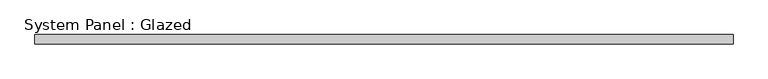
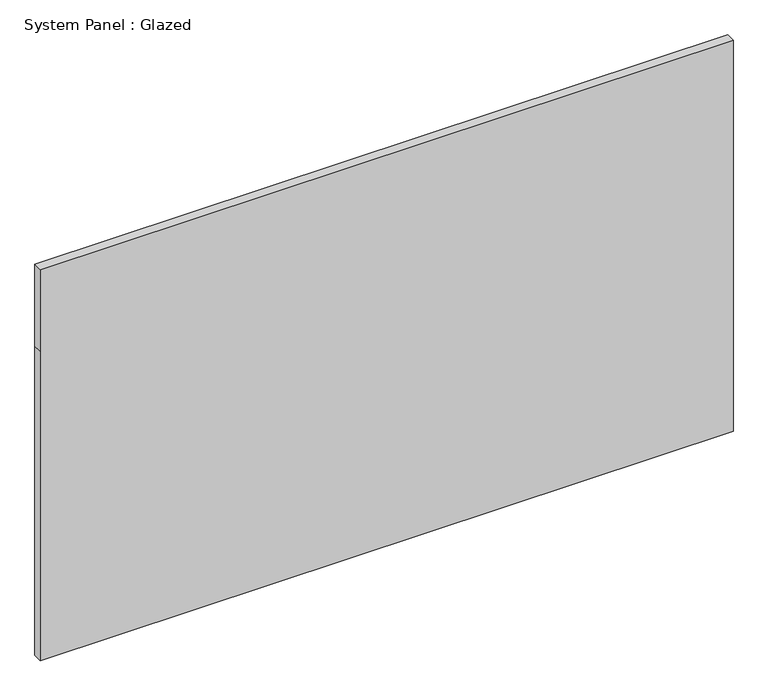
"""IFC4 building model written with IfcOpenShell, lengths in millimetres: plate geometry, System Panel : Glazed."""

import ifcopenshell
import ifcopenshell.guid

model = None  # the IFC model being written
_history = None  # IfcOwnerHistory: only IFC2X3 demands one
_inside = {}  # id of a spatial element -> (the spatial element, [elements in it])
_under = {}  # id of a project, library or spatial element -> (it, [spatial elements below it])
_declared = {}  # id of a project -> (the project, [libraries it declares])
_typed = {}  # id of a type object -> (the type object, [elements of that type])
_made_of = {}  # id of a material, layer set ... -> (it, [elements and type objects made of it])


def new_model(schema):
    """Start an empty IFC model of exactly this schema.

    Asked for "IFC4X3", IfcOpenShell would pick the latest addendum, in which some entities
    have other attributes; the version numbers below select the first issue.
    IFC2X3 requires an IfcOwnerHistory on every rooted entity: one is made here for all.
    """
    global model, _history
    if schema == "IFC4X3":
        model = ifcopenshell.file(schema_version=(4, 3, 0, 0))
    else:
        model = ifcopenshell.file(schema=schema)
    _inside.clear()
    _under.clear()
    _declared.clear()
    _typed.clear()
    _made_of.clear()
    _history = None
    if model.schema == "IFC2X3":
        org = make("IfcOrganization", Name="unknown")
        user = make(
            "IfcPersonAndOrganization",
            ThePerson=make("IfcPerson", FamilyName="unknown"),
            TheOrganization=org,
        )
        app = make(
            "IfcApplication",
            ApplicationDeveloper=org,
            Version="unknown",
            ApplicationFullName="unknown",
            ApplicationIdentifier="unknown",
        )
        _history = make(
            "IfcOwnerHistory",
            OwningUser=user,
            OwningApplication=app,
            ChangeAction="ADDED",
            CreationDate=0,
        )
    return model


def make(cls, **values):
    """One entity of the class cls with the attributes given. An attribute that is None is left unset."""
    return model.create_entity(
        cls, **{name: value for name, value in values.items() if value is not None}
    )


def rooted(cls, **values):
    """An entity with a GlobalId (a new one), such as an element, a storey or a relation."""
    return make(cls, GlobalId=ifcopenshell.guid.new(), OwnerHistory=_history, **values)


def si_unit(unit_type, name, prefix=None):
    """IfcSIUnit, for example si_unit("LENGTHUNIT", "METRE", prefix="MILLI")."""
    return make("IfcSIUnit", UnitType=unit_type, Prefix=prefix, Name=name)


def assignment(units):
    """IfcUnitAssignment: the units of a project."""
    return None if units is None else make("IfcUnitAssignment", Units=units)


def point(xyz):
    """IfcCartesianPoint."""
    return None if xyz is None else make("IfcCartesianPoint", Coordinates=xyz)


def direction(xyz):
    """IfcDirection."""
    return None if xyz is None else make("IfcDirection", DirectionRatios=xyz)


def frame(location, z_axis=None, x_axis=None):
    """IfcAxis2Placement3D, a coordinate frame: its origin and axes. An axis left out is left unset."""
    return make(
        "IfcAxis2Placement3D",
        Location=point(location),
        Axis=direction(z_axis),
        RefDirection=direction(x_axis),
    )


def origin():
    """The frame at (0, 0, 0) with its axes left unset."""
    return frame((0.0, 0.0, 0.0))


def place(relative_to, where):
    """IfcLocalPlacement: puts the frame where relative to a parent placement (None: the world)."""
    return make(
        "IfcLocalPlacement", PlacementRelTo=relative_to, RelativePlacement=where
    )


def context(
    kind, dimensions, precision=None, world=None, true_north=None, identifier=None
):
    """IfcGeometricRepresentationContext, for example the 3D "Model" context."""
    return make(
        "IfcGeometricRepresentationContext",
        ContextIdentifier=identifier,
        ContextType=kind,
        CoordinateSpaceDimension=dimensions,
        Precision=precision,
        WorldCoordinateSystem=world,
        TrueNorth=true_north,
    )


def project(units=None, contexts=None):
    """IfcProject with its units and contexts."""
    return rooted(
        "IfcProject",
        Name="project",
        RepresentationContexts=contexts,
        UnitsInContext=assignment(units),
    )


def spatial(cls, under=None, at=None, **own):
    """A site, building, storey or space (cls), placed at a placement, below another one or the project."""
    s = rooted(cls, ObjectPlacement=at, **own)
    if under is not None:
        _under.setdefault(under.id(), (under, []))[1].append(s)
    return s


def polyline(points):
    """IfcPolyline through the points."""
    return make("IfcPolyline", Points=[point(p) for p in points])


def outline(outer, holes=None, kind="AREA"):
    """IfcArbitraryClosedProfileDef: a profile drawn as a closed curve; with holes, ...WithVoids."""
    if holes is None:
        return make("IfcArbitraryClosedProfileDef", ProfileType=kind, OuterCurve=outer)
    return make(
        "IfcArbitraryProfileDefWithVoids",
        ProfileType=kind,
        OuterCurve=outer,
        InnerCurves=holes,
    )


def extrude(swept, where, along, depth):
    """IfcExtrudedAreaSolid: the profile swept, set in the frame where, extruded along a direction by depth."""
    return make(
        "IfcExtrudedAreaSolid",
        SweptArea=swept,
        Position=where,
        ExtrudedDirection=direction(along),
        Depth=depth,
    )


def shape(context_of_items, identifier, shape_type, items):
    """IfcShapeRepresentation: the items that make up one representation, for example the "Body"."""
    return make(
        "IfcShapeRepresentation",
        ContextOfItems=context_of_items,
        RepresentationIdentifier=identifier,
        RepresentationType=shape_type,
        Items=items,
    )


def source(mapping_origin, context_of_items, identifier, shape_type, items):
    """IfcRepresentationMap: a shape defined once, which mapped items show again and again."""
    return make(
        "IfcRepresentationMap",
        MappingOrigin=mapping_origin,
        MappedRepresentation=shape(context_of_items, identifier, shape_type, items),
    )


def transform(
    local_origin,
    x_axis=None,
    y_axis=None,
    z_axis=None,
    scale=None,
    scale2=None,
    scale3=None,
    uniform=True,
):
    """IfcCartesianTransformationOperator3D, or its non-uniform kind. x_axis, y_axis, z_axis: its Axis1, 2, 3."""
    if uniform:
        return make(
            "IfcCartesianTransformationOperator3D",
            Axis1=direction(x_axis),
            Axis2=direction(y_axis),
            LocalOrigin=point(local_origin),
            Scale=scale,
            Axis3=direction(z_axis),
        )
    return make(
        "IfcCartesianTransformationOperator3DnonUniform",
        Axis1=direction(x_axis),
        Axis2=direction(y_axis),
        LocalOrigin=point(local_origin),
        Scale=scale,
        Axis3=direction(z_axis),
        Scale2=scale2,
        Scale3=scale3,
    )


def mapped(mapping_source, mapping_target):
    """IfcMappedItem: shows the shape of a source again, moved by a transform."""
    return make(
        "IfcMappedItem", MappingSource=mapping_source, MappingTarget=mapping_target
    )


def made_of(thing, what):
    """Note that an element or type object is made of a material, layer set ...; save() writes the relation."""
    if what is not None:
        _made_of.setdefault(what.id(), (what, []))[1].append(thing)
    return thing


def element(
    cls,
    number,
    at=None,
    inside=None,
    cuts=None,
    type_object=None,
    material=None,
    context=None,
    identifier="Body",
    shape_type=None,
    held_by="IfcProductDefinitionShape",
    body=None,
    shapes=None,
    **own,
):
    """One element of the class cls, such as IfcWall. Its Tag is "e" and its number.

    at: its placement. inside: the storey or other place that contains it. cuts: it is an
    opening in that element (IfcRelVoidsElement). A single representation is given by context,
    identifier, shape_type and body (its items); several are given by shapes. held_by: the class
    of the entity that holds the representations. save() writes the other relations.
    """
    e = rooted(cls, Tag="e%d" % number, ObjectPlacement=at, **own)
    if body is not None:
        shapes = [shape(context, identifier, shape_type, body)]
    if shapes is not None:
        e.Representation = make(held_by, Representations=shapes)
    if inside is not None:
        _inside.setdefault(inside.id(), (inside, []))[1].append(e)
    if cuts is not None:
        rooted(
            "IfcRelVoidsElement", RelatingBuildingElement=cuts, RelatedOpeningElement=e
        )
    if type_object is not None:
        _typed.setdefault(type_object.id(), (type_object, []))[1].append(e)
    return made_of(e, material)


def aggregate(whole, parts):
    """IfcRelAggregates: a whole, such as a stair, and the parts it consists of."""
    return rooted("IfcRelAggregates", RelatingObject=whole, RelatedObjects=parts)


def save(model, path):
    """Write the relations noted so far, then the file.

    IfcRelAggregates (storeys below a building ...), IfcRelContainedInSpatialStructure (elements
    in a storey), IfcRelDefinesByType, IfcRelAssociatesMaterial and IfcRelDeclares: one each for
    every whole, place, type object, material and project.
    """
    for whole, parts in _under.values():
        aggregate(whole, parts)
    for where, things in _inside.values():
        rooted(
            "IfcRelContainedInSpatialStructure",
            RelatedElements=things,
            RelatingStructure=where,
        )
    for kind, things in _typed.values():
        rooted("IfcRelDefinesByType", RelatedObjects=things, RelatingType=kind)
    for what, things in _made_of.values():
        rooted("IfcRelAssociatesMaterial", RelatedObjects=things, RelatingMaterial=what)
    for by, libraries in _declared.values():
        rooted("IfcRelDeclares", RelatingContext=by, RelatedDefinitions=libraries)
    model.write(path)


def system_panel_glazed_d60e1f89(model_context):
    return source(origin(), model_context, "Body", "SweptSolid", [
        extrude(outline(polyline([(0.0, -968.375), (0.0, 968.375), (914.4, 968.375), (1155.7, 968.375), (1155.7, -968.375), (914.4, -968.375), (0.0, -968.375)])), frame((0.0, 19.05, 0.0), z_axis=(0.0, 1.0, 0.0), x_axis=(0.0, 0.0, 1.0)), (0.0, 0.0, 1.0), 25.4),
    ])


if __name__ == "__main__":
    model = new_model("IFC4")
    model_context = context("Model", 3, world=origin())
    ifc_project = project(units=[si_unit("LENGTHUNIT", "METRE", prefix="MILLI")], contexts=[model_context])
    site = spatial("IfcSite", under=ifc_project)
    building = spatial("IfcBuilding", under=site)
    placement = place(None, origin())
    system_panel_glazed_shape = system_panel_glazed_d60e1f89(model_context)
    element("IfcPlate", 1, ObjectType="System Panel : Glazed", at=placement, inside=building, context=model_context, shape_type="MappedRepresentation", body=[
        mapped(system_panel_glazed_shape, transform((0.0, 0.0, 0.0), x_axis=(1.0, 0.0, 0.0), y_axis=(0.0, 1.0, 0.0), z_axis=(0.0, 0.0, 1.0))),
    ])
    save(model, "model.ifc")

# Revit data of these elements
# Element 1 (IfcPlate, "System Panel : Glazed")
#   Materials on its faces: "Glass"
# Materials
#   "Glass": class "Glass", colour RGB 0 128 192, transparency 0.75
